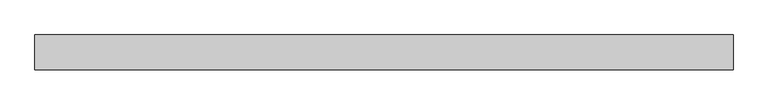
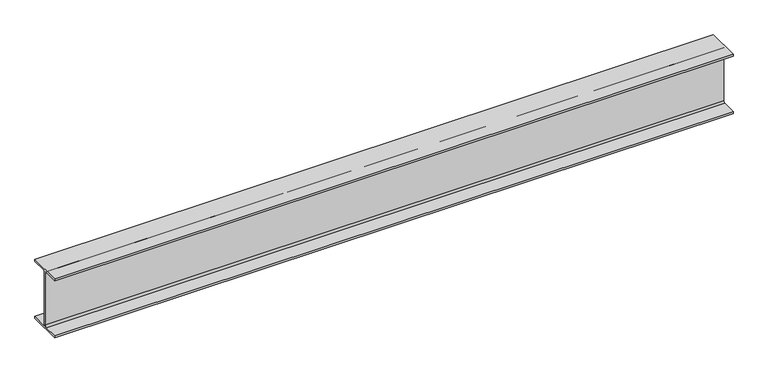
"""IFC4 building model written with IfcOpenShell, lengths in millimetres: beam geometry, Steel Beam_H-KSD3502 : H_SB_ASB_H-200x200x8x12."""

import ifcopenshell
import ifcopenshell.guid

model = None  # the IFC model being written
_history = None  # IfcOwnerHistory: only IFC2X3 demands one
_inside = {}  # id of a spatial element -> (the spatial element, [elements in it])
_under = {}  # id of a project, library or spatial element -> (it, [spatial elements below it])
_declared = {}  # id of a project -> (the project, [libraries it declares])
_typed = {}  # id of a type object -> (the type object, [elements of that type])
_made_of = {}  # id of a material, layer set ... -> (it, [elements and type objects made of it])


def new_model(schema):
    """Start an empty IFC model of exactly this schema.

    Asked for "IFC4X3", IfcOpenShell would pick the latest addendum, in which some entities
    have other attributes; the version numbers below select the first issue.
    IFC2X3 requires an IfcOwnerHistory on every rooted entity: one is made here for all.
    """
    global model, _history
    if schema == "IFC4X3":
        model = ifcopenshell.file(schema_version=(4, 3, 0, 0))
    else:
        model = ifcopenshell.file(schema=schema)
    _inside.clear()
    _under.clear()
    _declared.clear()
    _typed.clear()
    _made_of.clear()
    _history = None
    if model.schema == "IFC2X3":
        org = make("IfcOrganization", Name="unknown")
        user = make(
            "IfcPersonAndOrganization",
            ThePerson=make("IfcPerson", FamilyName="unknown"),
            TheOrganization=org,
        )
        app = make(
            "IfcApplication",
            ApplicationDeveloper=org,
            Version="unknown",
            ApplicationFullName="unknown",
            ApplicationIdentifier="unknown",
        )
        _history = make(
            "IfcOwnerHistory",
            OwningUser=user,
            OwningApplication=app,
            ChangeAction="ADDED",
            CreationDate=0,
        )
    return model


def make(cls, **values):
    """One entity of the class cls with the attributes given. An attribute that is None is left unset."""
    return model.create_entity(
        cls, **{name: value for name, value in values.items() if value is not None}
    )


def rooted(cls, **values):
    """An entity with a GlobalId (a new one), such as an element, a storey or a relation."""
    return make(cls, GlobalId=ifcopenshell.guid.new(), OwnerHistory=_history, **values)


def si_unit(unit_type, name, prefix=None):
    """IfcSIUnit, for example si_unit("LENGTHUNIT", "METRE", prefix="MILLI")."""
    return make("IfcSIUnit", UnitType=unit_type, Prefix=prefix, Name=name)


def assignment(units):
    """IfcUnitAssignment: the units of a project."""
    return None if units is None else make("IfcUnitAssignment", Units=units)


def point(xyz):
    """IfcCartesianPoint."""
    return None if xyz is None else make("IfcCartesianPoint", Coordinates=xyz)


def direction(xyz):
    """IfcDirection."""
    return None if xyz is None else make("IfcDirection", DirectionRatios=xyz)


def frame(location, z_axis=None, x_axis=None):
    """IfcAxis2Placement3D, a coordinate frame: its origin and axes. An axis left out is left unset."""
    return make(
        "IfcAxis2Placement3D",
        Location=point(location),
        Axis=direction(z_axis),
        RefDirection=direction(x_axis),
    )


def frame_2d(location, x_axis=None):
    """IfcAxis2Placement2D, a coordinate frame in the plane: its origin and x axis."""
    return make(
        "IfcAxis2Placement2D", Location=point(location), RefDirection=direction(x_axis)
    )


def origin():
    """The frame at (0, 0, 0) with its axes left unset."""
    return frame((0.0, 0.0, 0.0))


def place(relative_to, where):
    """IfcLocalPlacement: puts the frame where relative to a parent placement (None: the world)."""
    return make(
        "IfcLocalPlacement", PlacementRelTo=relative_to, RelativePlacement=where
    )


def context(
    kind, dimensions, precision=None, world=None, true_north=None, identifier=None
):
    """IfcGeometricRepresentationContext, for example the 3D "Model" context."""
    return make(
        "IfcGeometricRepresentationContext",
        ContextIdentifier=identifier,
        ContextType=kind,
        CoordinateSpaceDimension=dimensions,
        Precision=precision,
        WorldCoordinateSystem=world,
        TrueNorth=true_north,
    )


def project(units=None, contexts=None):
    """IfcProject with its units and contexts."""
    return rooted(
        "IfcProject",
        Name="project",
        RepresentationContexts=contexts,
        UnitsInContext=assignment(units),
    )


def spatial(cls, under=None, at=None, **own):
    """A site, building, storey or space (cls), placed at a placement, below another one or the project."""
    s = rooted(cls, ObjectPlacement=at, **own)
    if under is not None:
        _under.setdefault(under.id(), (under, []))[1].append(s)
    return s


def polyline(points):
    """IfcPolyline through the points."""
    return make("IfcPolyline", Points=[point(p) for p in points])


def circle_curve(where, radius):
    """IfcCircle in the frame where."""
    return make("IfcCircle", Position=where, Radius=radius)


def trimmed(basis, trim1, trim2, sense, master):
    """IfcTrimmedCurve: the piece of a basis curve between two trims."""
    return make(
        "IfcTrimmedCurve",
        BasisCurve=basis,
        Trim1=trim1,
        Trim2=trim2,
        SenseAgreement=sense,
        MasterRepresentation=master,
    )


def segment(curve, same_sense, transition):
    """IfcCompositeCurveSegment."""
    return make(
        "IfcCompositeCurveSegment",
        Transition=transition,
        SameSense=same_sense,
        ParentCurve=curve,
    )


def composite_curve(segments, self_intersect=None):
    """IfcCompositeCurve: segments joined end to end."""
    return make("IfcCompositeCurve", Segments=segments, SelfIntersect=self_intersect)


def outline(outer, holes=None, kind="AREA"):
    """IfcArbitraryClosedProfileDef: a profile drawn as a closed curve; with holes, ...WithVoids."""
    if holes is None:
        return make("IfcArbitraryClosedProfileDef", ProfileType=kind, OuterCurve=outer)
    return make(
        "IfcArbitraryProfileDefWithVoids",
        ProfileType=kind,
        OuterCurve=outer,
        InnerCurves=holes,
    )


def extrude(swept, where, along, depth):
    """IfcExtrudedAreaSolid: the profile swept, set in the frame where, extruded along a direction by depth."""
    return make(
        "IfcExtrudedAreaSolid",
        SweptArea=swept,
        Position=where,
        ExtrudedDirection=direction(along),
        Depth=depth,
    )


def shape(context_of_items, identifier, shape_type, items):
    """IfcShapeRepresentation: the items that make up one representation, for example the "Body"."""
    return make(
        "IfcShapeRepresentation",
        ContextOfItems=context_of_items,
        RepresentationIdentifier=identifier,
        RepresentationType=shape_type,
        Items=items,
    )


def source(mapping_origin, context_of_items, identifier, shape_type, items):
    """IfcRepresentationMap: a shape defined once, which mapped items show again and again."""
    return make(
        "IfcRepresentationMap",
        MappingOrigin=mapping_origin,
        MappedRepresentation=shape(context_of_items, identifier, shape_type, items),
    )


def transform(
    local_origin,
    x_axis=None,
    y_axis=None,
    z_axis=None,
    scale=None,
    scale2=None,
    scale3=None,
    uniform=True,
):
    """IfcCartesianTransformationOperator3D, or its non-uniform kind. x_axis, y_axis, z_axis: its Axis1, 2, 3."""
    if uniform:
        return make(
            "IfcCartesianTransformationOperator3D",
            Axis1=direction(x_axis),
            Axis2=direction(y_axis),
            LocalOrigin=point(local_origin),
            Scale=scale,
            Axis3=direction(z_axis),
        )
    return make(
        "IfcCartesianTransformationOperator3DnonUniform",
        Axis1=direction(x_axis),
        Axis2=direction(y_axis),
        LocalOrigin=point(local_origin),
        Scale=scale,
        Axis3=direction(z_axis),
        Scale2=scale2,
        Scale3=scale3,
    )


def mapped(mapping_source, mapping_target):
    """IfcMappedItem: shows the shape of a source again, moved by a transform."""
    return make(
        "IfcMappedItem", MappingSource=mapping_source, MappingTarget=mapping_target
    )


def made_of(thing, what):
    """Note that an element or type object is made of a material, layer set ...; save() writes the relation."""
    if what is not None:
        _made_of.setdefault(what.id(), (what, []))[1].append(thing)
    return thing


def element(
    cls,
    number,
    at=None,
    inside=None,
    cuts=None,
    type_object=None,
    material=None,
    context=None,
    identifier="Body",
    shape_type=None,
    held_by="IfcProductDefinitionShape",
    body=None,
    shapes=None,
    **own,
):
    """One element of the class cls, such as IfcWall. Its Tag is "e" and its number.

    at: its placement. inside: the storey or other place that contains it. cuts: it is an
    opening in that element (IfcRelVoidsElement). A single representation is given by context,
    identifier, shape_type and body (its items); several are given by shapes. held_by: the class
    of the entity that holds the representations. save() writes the other relations.
    """
    e = rooted(cls, Tag="e%d" % number, ObjectPlacement=at, **own)
    if body is not None:
        shapes = [shape(context, identifier, shape_type, body)]
    if shapes is not None:
        e.Representation = make(held_by, Representations=shapes)
    if inside is not None:
        _inside.setdefault(inside.id(), (inside, []))[1].append(e)
    if cuts is not None:
        rooted(
            "IfcRelVoidsElement", RelatingBuildingElement=cuts, RelatedOpeningElement=e
        )
    if type_object is not None:
        _typed.setdefault(type_object.id(), (type_object, []))[1].append(e)
    return made_of(e, material)


def aggregate(whole, parts):
    """IfcRelAggregates: a whole, such as a stair, and the parts it consists of."""
    return rooted("IfcRelAggregates", RelatingObject=whole, RelatedObjects=parts)


def save(model, path):
    """Write the relations noted so far, then the file.

    IfcRelAggregates (storeys below a building ...), IfcRelContainedInSpatialStructure (elements
    in a storey), IfcRelDefinesByType, IfcRelAssociatesMaterial and IfcRelDeclares: one each for
    every whole, place, type object, material and project.
    """
    for whole, parts in _under.values():
        aggregate(whole, parts)
    for where, things in _inside.values():
        rooted(
            "IfcRelContainedInSpatialStructure",
            RelatedElements=things,
            RelatingStructure=where,
        )
    for kind, things in _typed.values():
        rooted("IfcRelDefinesByType", RelatedObjects=things, RelatingType=kind)
    for what, things in _made_of.values():
        rooted("IfcRelAssociatesMaterial", RelatedObjects=things, RelatingMaterial=what)
    for by, libraries in _declared.values():
        rooted("IfcRelDeclares", RelatingContext=by, RelatedDefinitions=libraries)
    model.write(path)


def beam_561cba6f(model_context):
    return source(origin(), model_context, "Body", "SweptSolid", [
        extrude(outline(composite_curve([segment(polyline([(82.5, -141.5), (82.5, -151.7), (-82.5, -151.7), (-82.5, -141.5), (-11.9, -141.5)]), True, "CONTINUOUS"), segment(trimmed(circle_curve(frame_2d((-11.9, -132.6)), 8.9), [point((-11.9, -141.5))], [point((-3.0, -132.6))], True, "CARTESIAN"), True, "CONTINUOUS"), segment(polyline([(-3.0, -132.6), (-3.0, 132.6)]), True, "CONTINUOUS"), segment(trimmed(circle_curve(frame_2d((-11.9, 132.6)), 8.9), [point((-3.0, 132.6))], [point((-11.9, 141.5))], True, "CARTESIAN"), True, "CONTINUOUS"), segment(polyline([(-11.9, 141.5), (-82.5, 141.5), (-82.5, 151.7), (82.5, 151.7), (82.5, 141.5), (11.9, 141.5)]), True, "CONTINUOUS"), segment(trimmed(circle_curve(frame_2d((11.9, 132.6)), 8.9), [point((11.9, 141.5))], [point((3.0, 132.6))], True, "CARTESIAN"), True, "CONTINUOUS"), segment(polyline([(3.0, 132.6), (3.0, -132.6)]), True, "CONTINUOUS"), segment(trimmed(circle_curve(frame_2d((11.9, -132.6)), 8.9), [point((3.0, -132.6))], [point((11.9, -141.5))], True, "CARTESIAN"), True, "CONTINUOUS"), segment(polyline([(11.9, -141.5), (82.5, -141.5)]), True, "CONTINUOUS")], self_intersect=False)), frame((-1695.2828606, 0.0, 0.0), z_axis=(1.0, 0.0, 0.0), x_axis=(0.0, 1.0, 0.0)), (0.0, 0.0, 1.0), 3284.9531949),
    ])


if __name__ == "__main__":
    model = new_model("IFC4")
    model_context = context("Model", 3, world=origin())
    ifc_project = project(units=[si_unit("LENGTHUNIT", "METRE", prefix="MILLI")], contexts=[model_context])
    site = spatial("IfcSite", under=ifc_project)
    building = spatial("IfcBuilding", under=site)
    placement = place(None, origin())
    beam_shape = beam_561cba6f(model_context)
    element("IfcBeam", 1, ObjectType="Steel Beam_H-KSD3502 : H_SB_ASB_H-200x200x8x12", at=placement, inside=building, context=model_context, shape_type="MappedRepresentation", body=[
        mapped(beam_shape, transform((0.0, 0.0, 0.0), x_axis=(1.0, 0.0, 0.0), y_axis=(0.0, 1.0, 0.0), z_axis=(0.0, 0.0, 1.0))),
    ])
    save(model, "model.ifc")

# Revit data of these elements
# Type "Steel Beam_H-KSD3502 : H_SB_ASB_H-200x200x8x12"
#   Width = 20.0 cm
#   Web Thickness = 0.8 cm
#   Web Fillet = 1.3 cm
#   Warping Constant = 141376.0 cm⁶
#   Torsional Moment of Inertia = 26.2485 cm⁴
#   Torsional Modulus = 1.0 cm³
#   Section Area = 63.53 cm²
#   Plastic Modulus weak axis = 244.0 cm³
#   Plastic Modulus strong axis = 525.0 cm³
#   Perimeter = 1.16 m²/m
#   Nominal Weight = 49.90 kgf/m
#   Moment of Inertia weak axis = 1600.00 cm⁴
#   Moment of Inertia strong axis = 4720.00 cm⁴
#   Height = 20.0 cm
#   Flange Thickness = 1.2 cm
#   Elastic Modulus weak axis = 160.0 cm³
#   Elastic Modulus strong axis = 472.0 cm³
#   Centroid Vertical = 10.0 cm
#   Centroid Horizontal = 10.0 cm
#   Length [instance default] = 1.5240 m
#   Structural Material [instance default] = Steel, 45-345
#   Assembly Code = ""
# Element 1 (IfcBeam, "Steel Beam_H-KSD3502 : H_SB_ASB_H-200x200x8x12")
#   Structural Material = none
# Materials
#   "Steel, 45-345": class "Metal", colour RGB 189 187 185, transparency 0, Description = "Steel 345 MPa", Cost = 0
